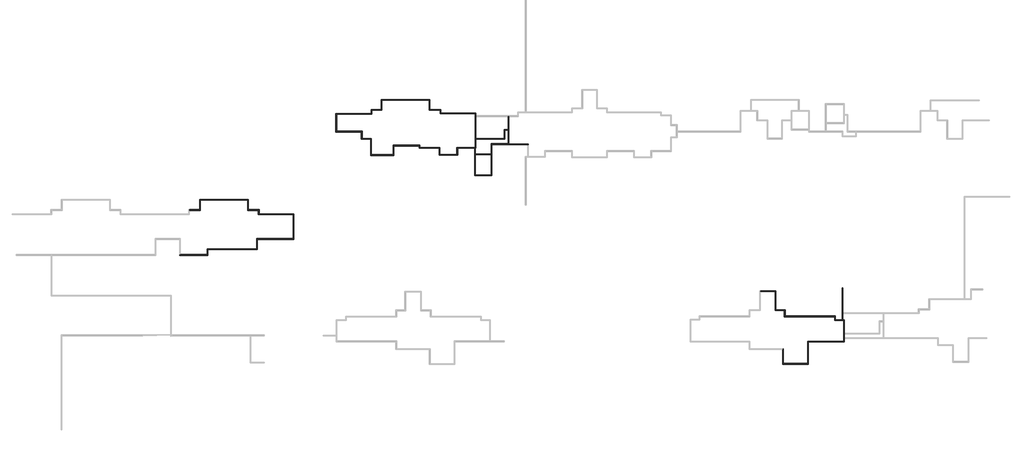
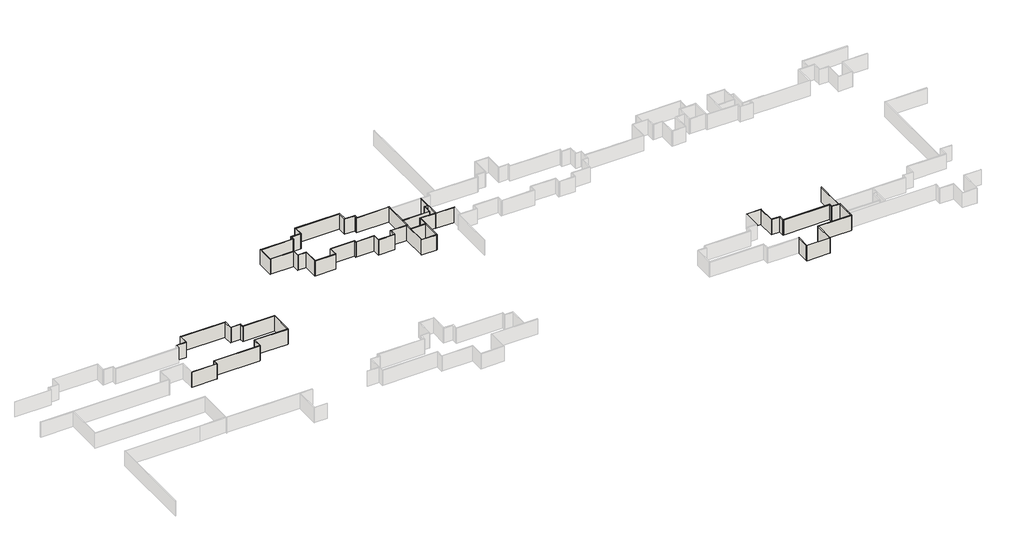
# One storey, part 3 of 8: 60 walls.
"""IFC4 building model written with IfcOpenShell, lengths in millimetres."""

import ifcopenshell
import ifcopenshell.guid

model = None  # the IFC model being written
_history = None  # IfcOwnerHistory: only IFC2X3 demands one
_inside = {}  # id of a spatial element -> (the spatial element, [elements in it])
_under = {}  # id of a project, library or spatial element -> (it, [spatial elements below it])
_declared = {}  # id of a project -> (the project, [libraries it declares])
_typed = {}  # id of a type object -> (the type object, [elements of that type])
_made_of = {}  # id of a material, layer set ... -> (it, [elements and type objects made of it])


def new_model(schema):
    """Start an empty IFC model of exactly this schema.

    Asked for "IFC4X3", IfcOpenShell would pick the latest addendum, in which some entities
    have other attributes; the version numbers below select the first issue.
    IFC2X3 requires an IfcOwnerHistory on every rooted entity: one is made here for all.
    """
    global model, _history
    if schema == "IFC4X3":
        model = ifcopenshell.file(schema_version=(4, 3, 0, 0))
    else:
        model = ifcopenshell.file(schema=schema)
    _inside.clear()
    _under.clear()
    _declared.clear()
    _typed.clear()
    _made_of.clear()
    _history = None
    if model.schema == "IFC2X3":
        org = make("IfcOrganization", Name="unknown")
        user = make(
            "IfcPersonAndOrganization",
            ThePerson=make("IfcPerson", FamilyName="unknown"),
            TheOrganization=org,
        )
        app = make(
            "IfcApplication",
            ApplicationDeveloper=org,
            Version="unknown",
            ApplicationFullName="unknown",
            ApplicationIdentifier="unknown",
        )
        _history = make(
            "IfcOwnerHistory",
            OwningUser=user,
            OwningApplication=app,
            ChangeAction="ADDED",
            CreationDate=0,
        )
    return model


def make(cls, **values):
    """One entity of the class cls with the attributes given. An attribute that is None is left unset."""
    return model.create_entity(
        cls, **{name: value for name, value in values.items() if value is not None}
    )


def rooted(cls, **values):
    """An entity with a GlobalId (a new one), such as an element, a storey or a relation."""
    return make(cls, GlobalId=ifcopenshell.guid.new(), OwnerHistory=_history, **values)


def si_unit(unit_type, name, prefix=None):
    """IfcSIUnit, for example si_unit("LENGTHUNIT", "METRE", prefix="MILLI")."""
    return make("IfcSIUnit", UnitType=unit_type, Prefix=prefix, Name=name)


def assignment(units):
    """IfcUnitAssignment: the units of a project."""
    return None if units is None else make("IfcUnitAssignment", Units=units)


def point(xyz):
    """IfcCartesianPoint."""
    return None if xyz is None else make("IfcCartesianPoint", Coordinates=xyz)


def direction(xyz):
    """IfcDirection."""
    return None if xyz is None else make("IfcDirection", DirectionRatios=xyz)


def frame(location, z_axis=None, x_axis=None):
    """IfcAxis2Placement3D, a coordinate frame: its origin and axes. An axis left out is left unset."""
    return make(
        "IfcAxis2Placement3D",
        Location=point(location),
        Axis=direction(z_axis),
        RefDirection=direction(x_axis),
    )


def origin():
    """The frame at (0, 0, 0) with its axes left unset."""
    return frame((0.0, 0.0, 0.0))


def origin_with_axes():
    """The frame at (0, 0, 0) with the z axis (0, 0, 1) and the x axis (1, 0, 0) written out."""
    return frame((0.0, 0.0, 0.0), z_axis=(0.0, 0.0, 1.0), x_axis=(1.0, 0.0, 0.0))


def place(relative_to, where):
    """IfcLocalPlacement: puts the frame where relative to a parent placement (None: the world)."""
    return make(
        "IfcLocalPlacement", PlacementRelTo=relative_to, RelativePlacement=where
    )


def context(
    kind, dimensions, precision=None, world=None, true_north=None, identifier=None
):
    """IfcGeometricRepresentationContext, for example the 3D "Model" context."""
    return make(
        "IfcGeometricRepresentationContext",
        ContextIdentifier=identifier,
        ContextType=kind,
        CoordinateSpaceDimension=dimensions,
        Precision=precision,
        WorldCoordinateSystem=world,
        TrueNorth=true_north,
    )


def project(units=None, contexts=None):
    """IfcProject with its units and contexts."""
    return rooted(
        "IfcProject",
        Name="project",
        RepresentationContexts=contexts,
        UnitsInContext=assignment(units),
    )


def spatial(cls, under=None, at=None, **own):
    """A site, building, storey or space (cls), placed at a placement, below another one or the project."""
    s = rooted(cls, ObjectPlacement=at, **own)
    if under is not None:
        _under.setdefault(under.id(), (under, []))[1].append(s)
    return s


def polyline(points):
    """IfcPolyline through the points."""
    return make("IfcPolyline", Points=[point(p) for p in points])


def outline(outer, holes=None, kind="AREA"):
    """IfcArbitraryClosedProfileDef: a profile drawn as a closed curve; with holes, ...WithVoids."""
    if holes is None:
        return make("IfcArbitraryClosedProfileDef", ProfileType=kind, OuterCurve=outer)
    return make(
        "IfcArbitraryProfileDefWithVoids",
        ProfileType=kind,
        OuterCurve=outer,
        InnerCurves=holes,
    )


def extrude(swept, where, along, depth):
    """IfcExtrudedAreaSolid: the profile swept, set in the frame where, extruded along a direction by depth."""
    return make(
        "IfcExtrudedAreaSolid",
        SweptArea=swept,
        Position=where,
        ExtrudedDirection=direction(along),
        Depth=depth,
    )


def faces_of(points, faces, orient=None, outer=None):
    """IfcFace entities. A face is a list of loops; a loop is a list of indices into points, from 0.

    orient and outer hold one flag for each loop. By default every Orientation is true, the
    first loop of a face is its IfcFaceOuterBound and the others are IfcFaceBound.
    """
    made = []
    for i, loops in enumerate(faces):
        bounds = []
        for j, loop in enumerate(loops):
            is_outer = j == 0 if outer is None else outer[i][j]
            bounds.append(
                make(
                    "IfcFaceOuterBound" if is_outer else "IfcFaceBound",
                    Bound=make("IfcPolyLoop", Polygon=[points[k] for k in loop]),
                    Orientation=True if orient is None else orient[i][j],
                )
            )
        made.append(make("IfcFace", Bounds=bounds))
    return made


def faceted_brep(points, faces, orient=None, outer=None, voids=None):
    """IfcFacetedBrep: a solid bounded by flat faces; with voids (closed shells), ...WithVoids."""
    shared = [point(p) for p in points]
    hull = make("IfcClosedShell", CfsFaces=faces_of(shared, faces, orient, outer))
    if voids is None:
        return make("IfcFacetedBrep", Outer=hull)
    return make(
        "IfcFacetedBrepWithVoids",
        Outer=hull,
        Voids=[
            make(cls, CfsFaces=faces_of(shared, fs, o, b)) for cls, fs, o, b in voids
        ],
    )


def shape(context_of_items, identifier, shape_type, items):
    """IfcShapeRepresentation: the items that make up one representation, for example the "Body"."""
    return make(
        "IfcShapeRepresentation",
        ContextOfItems=context_of_items,
        RepresentationIdentifier=identifier,
        RepresentationType=shape_type,
        Items=items,
    )


def made_of(thing, what):
    """Note that an element or type object is made of a material, layer set ...; save() writes the relation."""
    if what is not None:
        _made_of.setdefault(what.id(), (what, []))[1].append(thing)
    return thing


def element(
    cls,
    number,
    at=None,
    inside=None,
    cuts=None,
    type_object=None,
    material=None,
    context=None,
    identifier="Body",
    shape_type=None,
    held_by="IfcProductDefinitionShape",
    body=None,
    shapes=None,
    **own,
):
    """One element of the class cls, such as IfcWall. Its Tag is "e" and its number.

    at: its placement. inside: the storey or other place that contains it. cuts: it is an
    opening in that element (IfcRelVoidsElement). A single representation is given by context,
    identifier, shape_type and body (its items); several are given by shapes. held_by: the class
    of the entity that holds the representations. save() writes the other relations.
    """
    e = rooted(cls, Tag="e%d" % number, ObjectPlacement=at, **own)
    if body is not None:
        shapes = [shape(context, identifier, shape_type, body)]
    if shapes is not None:
        e.Representation = make(held_by, Representations=shapes)
    if inside is not None:
        _inside.setdefault(inside.id(), (inside, []))[1].append(e)
    if cuts is not None:
        rooted(
            "IfcRelVoidsElement", RelatingBuildingElement=cuts, RelatedOpeningElement=e
        )
    if type_object is not None:
        _typed.setdefault(type_object.id(), (type_object, []))[1].append(e)
    return made_of(e, material)


def aggregate(whole, parts):
    """IfcRelAggregates: a whole, such as a stair, and the parts it consists of."""
    return rooted("IfcRelAggregates", RelatingObject=whole, RelatedObjects=parts)


def save(model, path):
    """Write the relations noted so far, then the file.

    IfcRelAggregates (storeys below a building ...), IfcRelContainedInSpatialStructure (elements
    in a storey), IfcRelDefinesByType, IfcRelAssociatesMaterial and IfcRelDeclares: one each for
    every whole, place, type object, material and project.
    """
    for whole, parts in _under.values():
        aggregate(whole, parts)
    for where, things in _inside.values():
        rooted(
            "IfcRelContainedInSpatialStructure",
            RelatedElements=things,
            RelatingStructure=where,
        )
    for kind, things in _typed.values():
        rooted("IfcRelDefinesByType", RelatedObjects=things, RelatingType=kind)
    for what, things in _made_of.values():
        rooted("IfcRelAssociatesMaterial", RelatedObjects=things, RelatingMaterial=what)
    for by, libraries in _declared.values():
        rooted("IfcRelDeclares", RelatingContext=by, RelatedDefinitions=libraries)
    model.write(path)


model = new_model("IFC4")

# Units and contexts
model_context = context("Model", 3, world=origin())
ifc_project = project(units=[si_unit("LENGTHUNIT", "METRE", prefix="MILLI")], contexts=[model_context])

# Site, building, storey
site = spatial("IfcSite", under=ifc_project)
building = spatial("IfcBuilding", under=site)
storey = spatial("IfcBuildingStorey", under=building, Name="户型图", Elevation=0.0)

# Walls
placement = place(None, origin())
element("IfcWall", 1, ObjectType="所有墙体", at=placement, inside=storey, context=model_context, shape_type="Brep", body=[
    faceted_brep([(127910.0897862, 79520.2608397, 0.0), (129959.7629292, 79520.2608397, 0.0), (129959.7629292, 79520.2608397, 3300.0), (127910.0897862, 79520.2608397, 3300.0), (127910.0897862, 79640.2608397, 0.0), (127910.0897862, 79640.2608397, 3300.0), (129839.7629292, 79640.2608397, 3300.0), (129959.7629292, 79640.2608397, 3300.0), (129959.7629292, 79640.2608397, 0.0), (129839.7629292, 79640.2608397, 0.0)], [[[0, 1, 2, 3]], [[4, 5, 6, 7, 8, 9]], [[1, 0, 4, 9, 8]], [[3, 2, 7, 6, 5]], [[0, 3, 5, 4]], [[2, 1, 8, 7]]]),
])
element("IfcWall", 2, ObjectType="所有墙体", at=placement, inside=storey, context=model_context, shape_type="Brep", body=[
    faceted_brep([(129959.7629292, 79640.2608397, 0.0), (129959.7629292, 81522.3565617, 0.0), (129959.7629292, 81642.3565617, 0.0), (129959.7629292, 81642.3565617, 3300.0), (129959.7629292, 81522.3565617, 3300.0), (129959.7629292, 79640.2608397, 3300.0), (129839.7629292, 79640.2608397, 0.0), (129839.7629292, 79640.2608397, 3300.0), (129839.7629292, 81642.3565617, 3300.0), (129839.7629292, 81642.3565617, 0.0)], [[[0, 1, 2, 3, 4, 5]], [[6, 7, 8, 9]], [[2, 1, 0, 6, 9]], [[5, 4, 3, 8, 7]], [[0, 5, 7, 6]], [[3, 2, 9, 8]]]),
])
element("IfcWall", 3, ObjectType="所有墙体", at=placement, inside=storey, context=model_context, shape_type="Brep", body=[
    faceted_brep([(129959.7629292, 81522.3565617, 0.0), (139140.3371507, 81522.3565617, 0.0), (139260.3371507, 81522.3565617, 0.0), (139260.3371507, 81522.3565617, 3300.0), (139140.3371507, 81522.3565617, 3300.0), (129959.7629292, 81522.3565617, 3300.0), (129959.7629292, 81642.3565617, 0.0), (129959.7629292, 81642.3565617, 3300.0), (139260.3371507, 81642.3565617, 3300.0), (139260.3371507, 81642.3565617, 0.0)], [[[0, 1, 2, 3, 4, 5]], [[6, 7, 8, 9]], [[2, 1, 0, 6, 9]], [[5, 4, 3, 8, 7]], [[0, 5, 7, 6]], [[3, 2, 9, 8]]]),
])
element("IfcWall", 4, ObjectType="所有墙体", at=placement, inside=storey, context=model_context, shape_type="Brep", body=[
    faceted_brep([(139140.3371507, 81522.3565617, 0.0), (139140.3371507, 79520.2608397, 0.0), (139140.3371507, 79520.2608397, 3300.0), (139140.3371507, 81522.3565617, 3300.0), (139260.3371507, 81522.3565617, 0.0), (139260.3371507, 81522.3565617, 3300.0), (139260.3371507, 79640.2608397, 3300.0), (139260.3371507, 79520.2608397, 3300.0), (139260.3371507, 79520.2608397, 0.0), (139260.3371507, 79640.2608397, 0.0)], [[[0, 1, 2, 3]], [[4, 5, 6, 7, 8, 9]], [[1, 0, 4, 9, 8]], [[3, 2, 7, 6, 5]], [[0, 3, 5, 4]], [[2, 1, 8, 7]]]),
])
element("IfcWall", 5, ObjectType="所有墙体", at=placement, inside=storey, context=model_context, shape_type="Brep", body=[
    faceted_brep([(139260.3371507, 79520.2608397, 0.0), (141190.12079, 79520.2608397, 0.0), (141310.12079, 79520.2608397, 0.0), (141310.12079, 79520.2608397, 3300.0), (141190.12079, 79520.2608397, 3300.0), (139260.3371507, 79520.2608397, 3300.0), (139260.3371507, 79640.2608397, 0.0), (139260.3371507, 79640.2608397, 3300.0), (141310.12079, 79640.2608397, 3300.0), (141310.12079, 79640.2608397, 0.0)], [[[0, 1, 2, 3, 4, 5]], [[6, 7, 8, 9]], [[2, 1, 0, 6, 9]], [[5, 4, 3, 8, 7]], [[0, 5, 7, 6]], [[3, 2, 9, 8]]]),
])
element("IfcWall", 6, ObjectType="所有墙体", at=placement, inside=storey, context=model_context, shape_type="Brep", body=[
    faceted_brep([(141190.12079, 79520.2608397, 0.0), (141190.12079, 78721.1444171, 0.0), (141190.12079, 78721.1444171, 3300.0), (141190.12079, 79520.2608397, 3300.0), (141310.12079, 79520.2608397, 0.0), (141310.12079, 79520.2608397, 3300.0), (141310.12079, 78841.1444171, 3300.0), (141310.12079, 78721.1444171, 3300.0), (141310.12079, 78721.1444171, 0.0), (141310.12079, 78841.1444171, 0.0)], [[[0, 1, 2, 3]], [[4, 5, 6, 7, 8, 9]], [[1, 0, 4, 9, 8]], [[3, 2, 7, 6, 5]], [[0, 3, 5, 4]], [[2, 1, 8, 7]]]),
])
element("IfcWall", 7, ObjectType="所有墙体", at=placement, inside=storey, context=model_context, shape_type="Brep", body=[
    faceted_brep([(141310.12079, 78721.1444171, 0.0), (147870.12079, 78721.1444171, 0.0), (147990.12079, 78721.1444171, 0.0), (147990.12079, 78721.1444171, 3300.0), (147870.12079, 78721.1444171, 3300.0), (141310.12079, 78721.1444171, 3300.0), (141310.12079, 78841.1444171, 0.0), (141310.12079, 78841.1444171, 3300.0), (147990.12079, 78841.1444171, 3300.0), (147990.12079, 78841.1444171, 0.0)], [[[0, 1, 2, 3, 4, 5]], [[6, 7, 8, 9]], [[2, 1, 0, 6, 9]], [[5, 4, 3, 8, 7]], [[0, 5, 7, 6]], [[3, 2, 9, 8]]]),
])
element("IfcWall", 8, ObjectType="所有墙体", at=placement, inside=storey, context=model_context, shape_type="Brep", body=[
    faceted_brep([(147870.12079, 78721.1444171, 0.0), (147870.12079, 74052.1202767, 0.0), (147870.12079, 73932.1202767, 0.0), (147870.12079, 73932.1202767, 3300.0), (147870.12079, 74052.1202767, 3300.0), (147870.12079, 78721.1444171, 3300.0), (147990.12079, 78721.1444171, 0.0), (147990.12079, 78721.1444171, 3300.0), (147990.12079, 74052.1202767, 3300.0), (147990.12079, 73932.1202767, 3300.0), (147990.12079, 73932.1202767, 2700.0), (147990.12079, 73932.1202767, 0.0)], [[[0, 1, 2, 3, 4, 5]], [[6, 7, 8, 9, 10, 11]], [[2, 1, 0, 6, 11]], [[5, 4, 3, 9, 8, 7]], [[0, 5, 7, 6]], [[3, 2, 11, 10, 9]]]),
])
element("IfcWall", 9, ObjectType="所有墙体", at=placement, inside=storey, context=model_context, shape_type="Brep", body=[
    faceted_brep([(147870.12079, 74052.1202767, 0.0), (140890.165529, 74052.1202767, 0.0), (140890.165529, 74052.1202767, 3300.0), (147870.12079, 74052.1202767, 3300.0), (147870.12079, 73932.1202767, 0.0), (147870.12079, 73932.1202767, 3300.0), (141010.165529, 73932.1202767, 3300.0), (140890.165529, 73932.1202767, 3300.0), (140890.165529, 73932.1202767, 0.0), (141010.165529, 73932.1202767, 0.0)], [[[0, 1, 2, 3]], [[4, 5, 6, 7, 8, 9]], [[1, 0, 4, 9, 8]], [[3, 2, 7, 6, 5]], [[0, 3, 5, 4]], [[2, 1, 8, 7]]]),
])
element("IfcWall", 10, ObjectType="所有墙体", at=placement, inside=storey, context=model_context, shape_type="Brep", body=[
    faceted_brep([(140890.165529, 73932.1202767, 0.0), (140890.165529, 72052.4548583, 0.0), (140890.165529, 71932.4548583, 0.0), (140890.165529, 71932.4548583, 3300.0), (140890.165529, 72052.4548583, 3300.0), (140890.165529, 73932.1202767, 3300.0), (141010.165529, 73932.1202767, 0.0), (141010.165529, 73932.1202767, 3300.0), (141010.165529, 71932.4548583, 3300.0), (141010.165529, 71932.4548583, 0.0)], [[[0, 1, 2, 3, 4, 5]], [[6, 7, 8, 9]], [[2, 1, 0, 6, 9]], [[5, 4, 3, 8, 7]], [[0, 5, 7, 6]], [[3, 2, 9, 8]]]),
])
element("IfcWall", 11, ObjectType="所有墙体", at=placement, inside=storey, context=model_context, shape_type="Brep", body=[
    faceted_brep([(140890.165529, 72052.4548583, 0.0), (131290.162691, 72052.4548583, 0.0), (131290.162691, 72052.4548583, 3300.0), (140890.165529, 72052.4548583, 3300.0), (140890.165529, 71932.4548583, 0.0), (140890.165529, 71932.4548583, 3300.0), (131410.162691, 71932.4548583, 3300.0), (131290.162691, 71932.4548583, 3300.0), (131290.162691, 71932.4548583, 0.0), (131410.162691, 71932.4548583, 0.0)], [[[0, 1, 2, 3]], [[4, 5, 6, 7, 8, 9]], [[1, 0, 4, 9, 8]], [[3, 2, 7, 6, 5]], [[0, 3, 5, 4]], [[2, 1, 8, 7]]]),
])
element("IfcWall", 12, ObjectType="所有墙体", at=placement, inside=storey, context=model_context, shape_type="Brep", body=[
    faceted_brep([(131290.162691, 71932.4548583, 0.0), (131290.162691, 70952.1232979, 0.0), (131290.162691, 70832.1232979, 0.0), (131290.162691, 70832.1232979, 3300.0), (131290.162691, 70952.1232979, 3300.0), (131290.162691, 71932.4548583, 3300.0), (131410.162691, 71932.4548583, 0.0), (131410.162691, 71932.4548583, 3300.0), (131410.162691, 70832.1232979, 3300.0), (131410.162691, 70832.1232979, 0.0)], [[[0, 1, 2, 3, 4, 5]], [[6, 7, 8, 9]], [[2, 1, 0, 6, 9]], [[5, 4, 3, 8, 7]], [[0, 5, 7, 6]], [[3, 2, 9, 8]]]),
])
element("IfcWall", 13, ObjectType="所有墙体", at=placement, inside=storey, context=model_context, shape_type="Brep", body=[
    faceted_brep([(131290.162691, 70952.1232979, 0.0), (126110.2513394, 70952.1232979, 0.0), (125990.2513394, 70952.1232979, 0.0), (125990.2513394, 70952.1232979, 3300.0), (126110.2513394, 70952.1232979, 3300.0), (131290.162691, 70952.1232979, 3300.0), (131290.162691, 70832.1232979, 0.0), (131290.162691, 70832.1232979, 3300.0), (125990.2513394, 70832.1232979, 3300.0), (125990.2513394, 70832.1232979, 0.0)], [[[0, 1, 2, 3, 4, 5]], [[6, 7, 8, 9]], [[2, 1, 0, 6, 9]], [[5, 4, 3, 8, 7]], [[0, 5, 7, 6]], [[3, 2, 9, 8]]]),
])
element("IfcWall", 14, ObjectType="所有墙体", at=placement, inside=storey, context=model_context, shape_type="Brep", body=[
    faceted_brep([(189279.4180303, 97612.4890874, 0.0), (189279.4180303, 95102.0462442, 0.0), (189279.4180303, 94982.0462442, 0.0), (189279.4180303, 92353.7889647, 0.0), (189279.4180303, 92233.7889647, 0.0), (189279.4180303, 92173.7889647, 0.0), (189279.4180303, 92173.7889647, 3300.0), (189279.4180303, 92233.7889647, 3300.0), (189279.4180303, 92353.7889647, 3300.0), (189279.4180303, 94982.0462442, 3300.0), (189279.4180303, 95102.0462442, 3300.0), (189279.4180303, 97612.4890874, 3300.0), (189399.4180303, 97612.4890874, 0.0), (189399.4180303, 97612.4890874, 3300.0), (189399.4180303, 92293.7889647, 3300.0), (189399.4180303, 92173.7889647, 3300.0), (189399.4180303, 92173.7889647, 0.0), (189399.4180303, 92293.7889647, 0.0)], [[[0, 1, 2, 3, 4, 5, 6, 7, 8, 9, 10, 11]], [[12, 13, 14, 15, 16, 17]], [[5, 4, 3, 2, 1, 0, 12, 17, 16]], [[11, 10, 9, 8, 7, 6, 15, 14, 13]], [[6, 5, 16, 15]], [[0, 11, 13, 12]]]),
])
element("IfcWall", 15, ObjectType="所有墙体", at=placement, inside=storey, context=model_context, shape_type="Brep", body=[
    faceted_brep([(189399.4180303, 92173.7889647, 0.0), (193080.9640604, 92173.7889647, 0.0), (193200.9640604, 92173.7889647, 0.0), (193200.9640604, 92173.7889647, 3300.0), (193080.9640604, 92173.7889647, 3300.0), (189399.4180303, 92173.7889647, 3300.0), (189399.4180303, 92293.7889647, 0.0), (189399.4180303, 92293.7889647, 3300.0), (193200.9640604, 92293.7889647, 3300.0), (193200.9640604, 92293.7889647, 0.0)], [[[0, 1, 2, 3, 4, 5]], [[6, 7, 8, 9]], [[2, 1, 0, 6, 9]], [[5, 4, 3, 8, 7]], [[0, 5, 7, 6]], [[3, 2, 9, 8]]]),
])
element("IfcWall", 16, ObjectType="所有墙体", at=placement, inside=storey, context=model_context, shape_type="Brep", body=[
    faceted_brep([(156127.8219291, 98150.4331897, 0.0), (156127.8219291, 94631.7418551, 0.0), (156127.8219291, 94631.7418551, 3300.0), (156127.8219291, 97931.8352692, 3300.0), (156127.8219291, 98150.4331897, 3300.0), (156127.8219291, 98150.4331897, 2700.0), (156247.8219291, 98150.4331897, 0.0), (156247.8219291, 98150.4331897, 3300.0), (156247.8219291, 98030.4331897, 3300.0), (156247.8219291, 94751.7418551, 3300.0), (156247.8219291, 94631.7418551, 3300.0), (156247.8219291, 94631.7418551, 0.0), (156247.8219291, 94751.7418551, 0.0), (156247.8219291, 98030.4331897, 0.0), (156179.085005, 98150.4331897, 3300.0)], [[[0, 1, 2, 3, 4, 5]], [[6, 7, 8, 9, 10, 11, 12, 13]], [[1, 0, 6, 13, 12, 11]], [[4, 3, 2, 10, 9, 8, 7, 14]], [[2, 1, 11, 10]], [[0, 5, 4, 14, 7, 6]]]),
])
element("IfcWall", 17, ObjectType="所有墙体", at=placement, inside=storey, context=model_context, shape_type="Brep", body=[
    faceted_brep([(156247.8219291, 94631.7418551, 0.0), (161040.4072035, 94631.7418551, 0.0), (161160.4072035, 94631.7418551, 0.0), (161160.4072035, 94631.7418551, 3300.0), (161040.4072035, 94631.7418551, 3300.0), (156247.8219291, 94631.7418551, 3300.0), (156247.8219291, 94751.7418551, 0.0), (156247.8219291, 94751.7418551, 3300.0), (161160.4072035, 94751.7418551, 3300.0), (161160.4072035, 94751.7418551, 0.0)], [[[0, 1, 2, 3, 4, 5]], [[6, 7, 8, 9]], [[2, 1, 0, 6, 9]], [[5, 4, 3, 8, 7]], [[0, 5, 7, 6]], [[3, 2, 9, 8]]]),
])
element("IfcWall", 18, ObjectType="所有墙体", at=placement, inside=storey, context=model_context, shape_type="Brep", body=[
    faceted_brep([(161040.4072035, 94631.7418551, 0.0), (161040.4072035, 93231.7511932, 0.0), (161040.4072035, 93231.7511932, 3300.0), (161040.4072035, 94631.7418551, 3300.0), (161160.4072035, 94631.7418551, 0.0), (161160.4072035, 94631.7418551, 3300.0), (161160.4072035, 93351.7511932, 3300.0), (161160.4072035, 93231.7511932, 3300.0), (161160.4072035, 93231.7511932, 0.0), (161160.4072035, 93351.7511932, 0.0)], [[[0, 1, 2, 3]], [[4, 5, 6, 7, 8, 9]], [[1, 0, 4, 9, 8]], [[3, 2, 7, 6, 5]], [[0, 3, 5, 4]], [[2, 1, 8, 7]]]),
])
element("IfcWall", 19, ObjectType="所有墙体", at=placement, inside=storey, context=model_context, shape_type="Brep", body=[
    faceted_brep([(161160.4072035, 93231.7511932, 0.0), (162840.4072033, 93231.7511932, 0.0), (162960.4072033, 93231.7511932, 0.0), (162960.4072033, 93231.7511932, 3300.0), (162840.4072033, 93231.7511932, 3300.0), (161160.4072035, 93231.7511932, 3300.0), (161160.4072035, 93351.7511932, 0.0), (161160.4072035, 93351.7511932, 3300.0), (162960.4072033, 93351.7511932, 3300.0), (162960.4072033, 93351.7511932, 0.0)], [[[0, 1, 2, 3, 4, 5]], [[6, 7, 8, 9]], [[2, 1, 0, 6, 9]], [[5, 4, 3, 8, 7]], [[0, 5, 7, 6]], [[3, 2, 9, 8]]]),
])
element("IfcWall", 20, ObjectType="所有墙体", at=placement, inside=storey, context=model_context, shape_type="Brep", body=[
    faceted_brep([(162840.4072033, 93231.7511932, 0.0), (162840.4072033, 90105.9609607, 0.0), (162840.4072033, 90105.9609607, 3300.0), (162840.4072033, 93231.7511932, 3300.0), (162960.4072033, 93231.7511932, 0.0), (162960.4072033, 93231.7511932, 3300.0), (162960.4072033, 90225.9609607, 3300.0), (162960.4072033, 90105.9609607, 3300.0), (162960.4072033, 90105.9609607, 0.0), (162960.4072033, 90225.9609607, 0.0)], [[[0, 1, 2, 3]], [[4, 5, 6, 7, 8, 9]], [[1, 0, 4, 9, 8]], [[3, 2, 7, 6, 5]], [[0, 3, 5, 4]], [[2, 1, 8, 7]]]),
])
element("IfcWall", 21, ObjectType="所有墙体", at=placement, inside=storey, context=model_context, shape_type="Brep", body=[
    faceted_brep([(162960.4072033, 90105.9609607, 0.0), (167260.4072033, 90105.9609607, 0.0), (167260.4072033, 90105.9609607, 2700.0), (167260.4072033, 90105.9609607, 3300.0), (167100.4392887, 90105.9609607, 3300.0), (162960.4072033, 90105.9609607, 3300.0), (162960.4072033, 90225.9609607, 0.0), (162960.4072033, 90225.9609607, 3300.0), (167100.4392887, 90225.9609607, 3300.0), (167140.4072033, 90225.9609607, 3300.0), (167260.4072033, 90225.9609607, 3300.0), (167260.4072033, 90225.9609607, 0.0), (167140.4072033, 90225.9609607, 0.0)], [[[0, 1, 2, 3, 4, 5]], [[6, 7, 8, 9, 10, 11, 12]], [[1, 0, 6, 12, 11]], [[5, 4, 3, 10, 9, 8, 7]], [[0, 5, 7, 6]], [[3, 2, 1, 11, 10]]]),
])
element("IfcWall", 22, ObjectType="所有墙体", at=placement, inside=storey, context=model_context, shape_type="Brep", body=[
    faceted_brep([(167260.4072033, 90225.9609607, 0.0), (167260.4072033, 91931.7511932, 0.0), (167260.4072033, 92051.7511932, 0.0), (167260.4072033, 92051.7511932, 3300.0), (167260.4072033, 91931.7511932, 3300.0), (167260.4072033, 90341.7511932, 3300.0), (167260.4072033, 90225.9609607, 3300.0), (167140.4072033, 90225.9609607, 0.0), (167140.4072033, 90225.9609607, 2700.0), (167140.4072033, 90225.9609607, 3300.0), (167140.4072033, 90341.7511932, 3300.0), (167140.4072033, 92051.7511932, 3300.0), (167140.4072033, 92051.7511932, 0.0)], [[[0, 1, 2, 3, 4, 5, 6]], [[7, 8, 9, 10, 11, 12]], [[2, 1, 0, 7, 12]], [[6, 5, 4, 3, 11, 10, 9]], [[0, 6, 9, 8, 7]], [[3, 2, 12, 11]]]),
])
element("IfcWall", 23, ObjectType="所有墙体", at=placement, inside=storey, context=model_context, shape_type="Brep", body=[
    faceted_brep([(167260.4072033, 91931.7511932, 0.0), (172190.4075168, 91931.7511932, 0.0), (172310.4075168, 91931.7511932, 0.0), (172310.4075168, 91931.7511932, 3300.0), (172190.4075168, 91931.7511932, 3300.0), (167260.4072033, 91931.7511932, 3300.0), (167260.4072033, 92051.7511932, 0.0), (167260.4072033, 92051.7511932, 3300.0), (172310.4075168, 92051.7511932, 3300.0), (172310.4075168, 92051.7511932, 0.0)], [[[0, 1, 2, 3, 4, 5]], [[6, 7, 8, 9]], [[2, 1, 0, 6, 9]], [[5, 4, 3, 8, 7]], [[0, 5, 7, 6]], [[3, 2, 9, 8]]]),
])
element("IfcWall", 24, ObjectType="所有墙体", at=placement, inside=storey, context=model_context, shape_type="Brep", body=[
    faceted_brep([(172190.4075168, 91931.7511932, 0.0), (172190.4075168, 91531.3826392, 0.0), (172190.4075168, 91531.3826392, 3300.0), (172190.4075168, 91931.7511932, 3300.0), (172310.4075168, 91931.7511932, 0.0), (172310.4075168, 91931.7511932, 3300.0), (172310.4075168, 91651.3826392, 3300.0), (172310.4075168, 91531.3826392, 3300.0), (172310.4075168, 91531.3826392, 0.0), (172310.4075168, 91651.3826392, 0.0)], [[[0, 1, 2, 3]], [[4, 5, 6, 7, 8, 9]], [[1, 0, 4, 9, 8]], [[3, 2, 7, 6, 5]], [[0, 3, 5, 4]], [[2, 1, 8, 7]]]),
])
element("IfcWall", 25, ObjectType="所有墙体", at=placement, inside=storey, context=model_context, shape_type="Brep", body=[
    faceted_brep([(172310.4075168, 91531.3826392, 0.0), (176040.4072033, 91531.3826392, 0.0), (176160.4072033, 91531.3826392, 0.0), (176160.4072033, 91531.3826392, 3300.0), (176040.4072033, 91531.3826392, 3300.0), (172310.4075168, 91531.3826392, 3300.0), (172310.4075168, 91651.3826392, 0.0), (172310.4075168, 91651.3826392, 3300.0), (176160.4072033, 91651.3826392, 3300.0), (176160.4072033, 91651.3826392, 0.0)], [[[0, 1, 2, 3, 4, 5]], [[6, 7, 8, 9]], [[2, 1, 0, 6, 9]], [[5, 4, 3, 8, 7]], [[0, 5, 7, 6]], [[3, 2, 9, 8]]]),
])
element("IfcWall", 26, ObjectType="所有墙体", at=placement, inside=storey, context=model_context, shape_type="Brep", body=[
    faceted_brep([(176040.4072033, 91531.3826392, 0.0), (176040.4072033, 90131.7511932, 0.0), (176040.4072033, 90131.7511932, 3300.0), (176040.4072033, 91531.3826392, 3300.0), (176160.4072033, 91531.3826392, 0.0), (176160.4072033, 91531.3826392, 3300.0), (176160.4072033, 90251.7511932, 3300.0), (176160.4072033, 90131.7511932, 3300.0), (176160.4072033, 90131.7511932, 0.0), (176160.4072033, 90251.7511932, 0.0)], [[[0, 1, 2, 3]], [[4, 5, 6, 7, 8, 9]], [[1, 0, 4, 9, 8]], [[3, 2, 7, 6, 5]], [[0, 3, 5, 4]], [[2, 1, 8, 7]]]),
])
element("IfcWall", 27, ObjectType="所有墙体", at=placement, inside=storey, context=model_context, shape_type="Brep", body=[
    faceted_brep([(176160.4072033, 90131.7511932, 0.0), (179560.4072033, 90131.7511932, 0.0), (179560.4072033, 90131.7511932, 3300.0), (176160.4072033, 90131.7511932, 3300.0), (176160.4072033, 90251.7511932, 0.0), (176160.4072033, 90251.7511932, 3300.0), (179440.4072033, 90251.7511932, 3300.0), (179560.4072033, 90251.7511932, 3300.0), (179560.4072033, 90251.7511932, 0.0), (179440.4072033, 90251.7511932, 0.0)], [[[0, 1, 2, 3]], [[4, 5, 6, 7, 8, 9]], [[1, 0, 4, 9, 8]], [[3, 2, 7, 6, 5]], [[0, 3, 5, 4]], [[2, 1, 8, 7]]]),
])
element("IfcWall", 28, ObjectType="所有墙体", at=placement, inside=storey, context=model_context, shape_type="Brep", body=[
    faceted_brep([(179560.4072033, 90251.7511932, 0.0), (179560.4072033, 91531.3826392, 0.0), (179560.4072033, 91651.3826392, 0.0), (179560.4072033, 91651.3826392, 3300.0), (179560.4072033, 91531.3826392, 3300.0), (179560.4072033, 90251.7511932, 3300.0), (179440.4072033, 90251.7511932, 0.0), (179440.4072033, 90251.7511932, 3300.0), (179440.4072033, 91651.3826392, 3300.0), (179440.4072033, 91651.3826392, 0.0)], [[[0, 1, 2, 3, 4, 5]], [[6, 7, 8, 9]], [[2, 1, 0, 6, 9]], [[5, 4, 3, 8, 7]], [[0, 5, 7, 6]], [[3, 2, 9, 8]]]),
])
element("IfcWall", 29, ObjectType="所有墙体", at=placement, inside=storey, context=model_context, shape_type="Brep", body=[
    faceted_brep([(179560.4072033, 91531.3826392, 0.0), (182840.4077224, 91531.3826392, 0.0), (182960.4077224, 91531.3826392, 0.0), (183060.4077201, 91531.3826392, 0.0), (183060.4077201, 91531.3826392, 3300.0), (182960.4077224, 91531.3826392, 3300.0), (182840.4077224, 91531.3826392, 3300.0), (179560.4072033, 91531.3826392, 3300.0), (179560.4072033, 91651.3826392, 0.0), (179560.4072033, 91651.3826392, 3300.0), (182940.4077201, 91651.3826392, 3300.0), (183060.4077201, 91651.3826392, 3300.0), (183060.4077201, 91651.3826392, 0.0), (182940.4077201, 91651.3826392, 0.0)], [[[0, 1, 2, 3, 4, 5, 6, 7]], [[8, 9, 10, 11, 12, 13]], [[3, 2, 1, 0, 8, 13, 12]], [[7, 6, 5, 4, 11, 10, 9]], [[0, 7, 9, 8]], [[4, 3, 12, 11]]]),
])
element("IfcWall", 30, ObjectType="所有墙体", at=placement, inside=storey, context=model_context, shape_type="Brep", body=[
    faceted_brep([(183060.4077201, 91651.3826392, 0.0), (183060.4077201, 93231.7450908, 0.0), (183060.4077201, 93351.7450908, 0.0), (183060.4077201, 97612.4890874, 0.0), (183060.4077201, 97732.4890874, 0.0), (183060.4077201, 98250.4331897, 0.0), (183060.4077201, 98250.4331897, 3300.0), (183060.4077201, 97732.4890874, 3300.0), (183060.4077201, 97612.4890874, 3300.0), (183060.4077201, 93351.7450908, 3300.0), (183060.4077201, 93231.7450908, 3300.0), (183060.4077201, 91651.3826392, 3300.0), (182940.4077201, 91651.3826392, 0.0), (182940.4077201, 91651.3826392, 3300.0), (182940.4077201, 98130.4331897, 3300.0), (182940.4077201, 98250.4331897, 3300.0), (182940.4077201, 98250.4331897, 0.0), (182940.4077201, 98130.4331897, 0.0)], [[[0, 1, 2, 3, 4, 5, 6, 7, 8, 9, 10, 11]], [[12, 13, 14, 15, 16, 17]], [[5, 4, 3, 2, 1, 0, 12, 17, 16]], [[11, 10, 9, 8, 7, 6, 15, 14, 13]], [[0, 11, 13, 12]], [[6, 5, 16, 15]]]),
])
element("IfcWall", 31, ObjectType="所有墙体", at=placement, inside=storey, context=model_context, shape_type="Brep", body=[
    faceted_brep([(182940.4077201, 98250.4331897, 0.0), (176349.86269, 98250.4331897, 0.0), (176229.86269, 98250.4331897, 0.0), (176229.86269, 98250.4331897, 3300.0), (176349.86269, 98250.4331897, 3300.0), (182940.4077201, 98250.4331897, 3300.0), (182940.4077201, 98130.4331897, 0.0), (182940.4077201, 98130.4331897, 3300.0), (176229.86269, 98130.4331897, 3300.0), (176229.86269, 98130.4331897, 0.0)], [[[0, 1, 2, 3, 4, 5]], [[6, 7, 8, 9]], [[2, 1, 0, 6, 9]], [[5, 4, 3, 8, 7]], [[0, 5, 7, 6]], [[3, 2, 9, 8]]]),
])
element("IfcWall", 32, ObjectType="所有墙体", at=placement, inside=storey, context=model_context, shape_type="Brep", body=[
    faceted_brep([(176349.86269, 98250.4331897, 0.0), (176349.86269, 98950.4331897, 0.0), (176349.86269, 98950.4331897, 3300.0), (176349.86269, 98250.4331897, 3300.0), (176229.86269, 98250.4331897, 0.0), (176229.86269, 98250.4331897, 3300.0), (176229.86269, 98830.4331897, 3300.0), (176229.86269, 98950.4331897, 3300.0), (176229.86269, 98950.4331897, 0.0), (176229.86269, 98830.4331897, 0.0)], [[[0, 1, 2, 3]], [[4, 5, 6, 7, 8, 9]], [[1, 0, 4, 9, 8]], [[3, 2, 7, 6, 5]], [[0, 3, 5, 4]], [[2, 1, 8, 7]]]),
])
element("IfcWall", 33, ObjectType="所有墙体", at=placement, inside=storey, context=model_context, shape_type="Brep", body=[
    faceted_brep([(176229.86269, 98950.4331897, 0.0), (174249.8870953, 98950.4331897, 0.0), (174129.8870953, 98950.4331897, 0.0), (174129.8870953, 98950.4331897, 3300.0), (174249.8870953, 98950.4331897, 3300.0), (176229.86269, 98950.4331897, 3300.0), (176229.86269, 98830.4331897, 0.0), (176229.86269, 98830.4331897, 3300.0), (174129.8870953, 98830.4331897, 3300.0), (174129.8870953, 98830.4331897, 0.0)], [[[0, 1, 2, 3, 4, 5]], [[6, 7, 8, 9]], [[2, 1, 0, 6, 9]], [[5, 4, 3, 8, 7]], [[0, 5, 7, 6]], [[3, 2, 9, 8]]]),
])
element("IfcWall", 34, ObjectType="所有墙体", at=placement, inside=storey, context=model_context, shape_type="Brep", body=[
    faceted_brep([(174249.8870953, 98950.4331897, 0.0), (174249.8870953, 100902.3018651, 0.0), (174249.8870953, 100902.3018651, 3300.0), (174249.8870953, 98950.4331897, 3300.0), (174129.8870953, 98950.4331897, 0.0), (174129.8870953, 98950.4331897, 3300.0), (174129.8870953, 100782.3018651, 3300.0), (174129.8870953, 100902.3018651, 3300.0), (174129.8870953, 100902.3018651, 0.0), (174129.8870953, 100782.3018651, 0.0)], [[[0, 1, 2, 3]], [[4, 5, 6, 7, 8, 9]], [[1, 0, 4, 9, 8]], [[3, 2, 7, 6, 5]], [[0, 3, 5, 4]], [[2, 1, 8, 7]]]),
])
element("IfcWall", 35, ObjectType="所有墙体", at=placement, inside=storey, context=model_context, shape_type="Brep", body=[
    faceted_brep([(174129.8870953, 100902.3018651, 0.0), (164879.9002964, 100902.3018651, 0.0), (164879.9002964, 100902.3018651, 3300.0), (174129.8870953, 100902.3018651, 3300.0), (174129.8870953, 100782.3018651, 0.0), (174129.8870953, 100782.3018651, 3300.0), (164999.9002964, 100782.3018651, 3300.0), (164879.9002964, 100782.3018651, 3300.0), (164879.9002964, 100782.3018651, 0.0), (164999.9002964, 100782.3018651, 0.0)], [[[0, 1, 2, 3]], [[4, 5, 6, 7, 8, 9]], [[1, 0, 4, 9, 8]], [[3, 2, 7, 6, 5]], [[0, 3, 5, 4]], [[2, 1, 8, 7]]]),
])
element("IfcWall", 36, ObjectType="所有墙体", at=placement, inside=storey, context=model_context, shape_type="Brep", body=[
    faceted_brep([(164879.9002964, 100782.3018651, 0.0), (164879.9002964, 98950.4331897, 0.0), (164879.9002964, 98830.4331897, 0.0), (164879.9002964, 98830.4331897, 3300.0), (164879.9002964, 98950.4331897, 3300.0), (164879.9002964, 100782.3018651, 3300.0), (164999.9002964, 100782.3018651, 0.0), (164999.9002964, 100782.3018651, 3300.0), (164999.9002964, 98830.4331897, 3300.0), (164999.9002964, 98830.4331897, 0.0)], [[[0, 1, 2, 3, 4, 5]], [[6, 7, 8, 9]], [[2, 1, 0, 6, 9]], [[5, 4, 3, 8, 7]], [[0, 5, 7, 6]], [[3, 2, 9, 8]]]),
])
element("IfcWall", 37, ObjectType="所有墙体", at=placement, inside=storey, context=model_context, shape_type="Brep", body=[
    faceted_brep([(164879.9002964, 98950.4331897, 0.0), (162917.5304809, 98950.4331897, 0.0), (162917.5304809, 98950.4331897, 3300.0), (164879.9002964, 98950.4331897, 3300.0), (164879.9002964, 98830.4331897, 0.0), (164879.9002964, 98830.4331897, 3300.0), (163037.5304809, 98830.4331897, 3300.0), (162917.5304809, 98830.4331897, 3300.0), (162917.5304809, 98830.4331897, 0.0), (163037.5304809, 98830.4331897, 0.0)], [[[0, 1, 2, 3]], [[4, 5, 6, 7, 8, 9]], [[1, 0, 4, 9, 8]], [[3, 2, 7, 6, 5]], [[0, 3, 5, 4]], [[2, 1, 8, 7]]]),
])
element("IfcWall", 38, ObjectType="所有墙体", at=placement, inside=storey, context=model_context, shape_type="Brep", body=[
    faceted_brep([(162917.5304809, 98830.4331897, 0.0), (162917.5304809, 98150.4331897, 0.0), (162917.5304809, 98030.4331897, 0.0), (162917.5304809, 98030.4331897, 3300.0), (162917.5304809, 98150.4331897, 3300.0), (162917.5304809, 98830.4331897, 3300.0), (163037.5304809, 98830.4331897, 0.0), (163037.5304809, 98830.4331897, 3300.0), (163037.5304809, 98030.4331897, 3300.0), (163037.5304809, 98030.4331897, 0.0)], [[[0, 1, 2, 3, 4, 5]], [[6, 7, 8, 9]], [[2, 1, 0, 6, 9]], [[5, 4, 3, 8, 7]], [[0, 5, 7, 6]], [[3, 2, 9, 8]]]),
])
element("IfcWall", 39, ObjectType="所有墙体", at=placement, inside=storey, context=model_context, shape_type="SweptSolid", body=[
    extrude(outline(polyline([(156247.8219291, 98150.4331897), (162917.5304809, 98150.4331897), (162917.5304809, 98030.4331897), (156247.8219291, 98030.4331897), (156247.8219291, 98150.4331897)])), origin_with_axes(), (0.0, 0.0, 1.0), 3300.0),
])
element("IfcWall", 40, ObjectType="所有墙体", at=placement, inside=storey, context=model_context, shape_type="Brep", body=[
    faceted_brep([(189279.4180303, 95102.0462442, 0.0), (188540.4072025, 95102.0462442, 0.0), (188540.4072025, 95102.0462442, 3300.0), (189279.4180303, 95102.0462442, 3300.0), (189279.4180303, 94982.0462442, 0.0), (189279.4180303, 94982.0462442, 3300.0), (188660.4072025, 94982.0462442, 3300.0), (188540.4072025, 94982.0462442, 3300.0), (188540.4072025, 94982.0462442, 0.0), (188660.4072025, 94982.0462442, 0.0)], [[[0, 1, 2, 3]], [[4, 5, 6, 7, 8, 9]], [[1, 0, 4, 9, 8]], [[3, 2, 7, 6, 5]], [[0, 3, 5, 4]], [[2, 1, 8, 7]]]),
])
element("IfcWall", 41, ObjectType="所有墙体", at=placement, inside=storey, context=model_context, shape_type="Brep", body=[
    faceted_brep([(188540.4072025, 94982.0462442, 0.0), (188540.4072025, 93351.7450908, 0.0), (188540.4072025, 93231.7450908, 0.0), (188540.4072025, 93231.7450908, 3300.0), (188540.4072025, 93351.7450908, 3300.0), (188540.4072025, 94982.0462442, 3300.0), (188660.4072025, 94982.0462442, 0.0), (188660.4072025, 94982.0462442, 3300.0), (188660.4072025, 93231.7450908, 3300.0), (188660.4072025, 93231.7450908, 0.0)], [[[0, 1, 2, 3, 4, 5]], [[6, 7, 8, 9]], [[2, 1, 0, 6, 9]], [[5, 4, 3, 8, 7]], [[0, 5, 7, 6]], [[3, 2, 9, 8]]]),
])
element("IfcWall", 42, ObjectType="所有墙体", at=placement, inside=storey, context=model_context, shape_type="SweptSolid", body=[
    extrude(outline(polyline([(183060.4077201, 93351.7450908), (188540.4072025, 93351.7450908), (188540.4072025, 93231.7450908), (183060.4077201, 93231.7450908), (183060.4077201, 93351.7450908)])), origin_with_axes(), (0.0, 0.0, 1.0), 3300.0),
])
element("IfcWall", 43, ObjectType="所有墙体", at=placement, inside=storey, context=model_context, shape_type="Brep", body=[
    faceted_brep([(182840.4077224, 91531.3826392, 0.0), (182840.4077224, 86352.1684203, 0.0), (182840.4077224, 86352.1684203, 3300.0), (182840.4077224, 91531.3826392, 3300.0), (182960.4077224, 91531.3826392, 0.0), (182960.4077224, 91531.3826392, 3300.0), (182960.4077224, 90351.743349, 3300.0), (182960.4077224, 90231.743349, 3300.0), (182960.4077224, 86352.1684203, 3300.0), (182960.4077224, 86352.1684203, 0.0), (182960.4077224, 90231.743349, 0.0), (182960.4077224, 90351.743349, 0.0)], [[[0, 1, 2, 3]], [[4, 5, 6, 7, 8, 9, 10, 11]], [[1, 0, 4, 11, 10, 9]], [[3, 2, 8, 7, 6, 5]], [[0, 3, 5, 4]], [[2, 1, 9, 8]]]),
])
element("IfcWall", 44, ObjectType="所有墙体", at=placement, inside=storey, context=model_context, shape_type="SweptSolid", body=[
    extrude(outline(polyline([(186040.4077224, 90231.743349), (182960.4077224, 90231.743349), (182960.4077224, 90351.743349), (186040.4077224, 90351.743349), (186040.4077224, 90231.743349)])), origin_with_axes(), (0.0, 0.0, 1.0), 3300.0),
])
element("IfcWall", 45, ObjectType="所有墙体", at=placement, inside=storey, context=model_context, shape_type="Brep", body=[
    faceted_brep([(186040.4077224, 92233.7889647, 0.0), (186040.4077224, 90351.743349, 0.0), (186040.4077224, 90231.743349, 0.0), (186040.4077224, 86352.1684203, 0.0), (186040.4077224, 86232.1684203, 0.0), (186040.4077224, 86232.1684203, 3300.0), (186040.4077224, 86352.1684203, 3300.0), (186040.4077224, 86381.1826239, 3300.0), (186040.4077224, 86681.1826239, 3300.0), (186040.4077224, 90231.743349, 3300.0), (186040.4077224, 90351.743349, 3300.0), (186040.4077224, 92233.7889647, 3300.0), (186160.4077224, 92233.7889647, 0.0), (186160.4077224, 92233.7889647, 3300.0), (186160.4077224, 86681.1826239, 3300.0), (186160.4077224, 86381.1826239, 3300.0), (186160.4077224, 86232.1684203, 3300.0), (186160.4077224, 86232.1684203, 0.0)], [[[0, 1, 2, 3, 4, 5, 6, 7, 8, 9, 10, 11]], [[12, 13, 14, 15, 16, 17]], [[4, 3, 2, 1, 0, 12, 17]], [[11, 10, 9, 8, 7, 6, 5, 16, 15, 14, 13]], [[5, 4, 17, 16]], [[0, 11, 13, 12]]]),
])
element("IfcWall", 46, ObjectType="所有墙体", at=placement, inside=storey, context=model_context, shape_type="Brep", body=[
    faceted_brep([(186040.4077224, 86352.1684203, 0.0), (182960.4077224, 86352.1684203, 0.0), (182840.4077224, 86352.1684203, 0.0), (182840.4077224, 86352.1684203, 3300.0), (182960.4077224, 86352.1684203, 3300.0), (183014.313141, 86352.1684203, 3300.0), (186040.4077224, 86352.1684203, 3300.0), (186040.4077224, 86232.1684203, 0.0), (186040.4077224, 86232.1684203, 3300.0), (183054.7628482, 86232.1684203, 3300.0), (182840.4077224, 86232.1684203, 3300.0), (182840.4077224, 86232.1684203, 2700.0), (182840.4077224, 86232.1684203, 0.0)], [[[0, 1, 2, 3, 4, 5, 6]], [[7, 8, 9, 10, 11, 12]], [[2, 1, 0, 7, 12]], [[6, 5, 4, 3, 10, 9, 8]], [[0, 6, 8, 7]], [[3, 2, 12, 11, 10]]]),
])
element("IfcWall", 47, ObjectType="所有墙体", at=placement, inside=storey, context=model_context, shape_type="Brep", body=[
    faceted_brep([(189279.4180303, 92353.7889647, 0.0), (186039.4180303, 92353.7889647, 0.0), (186039.4180303, 92353.7889647, 3300.0), (189279.4180303, 92353.7889647, 3300.0), (189279.4180303, 92233.7889647, 0.0), (189279.4180303, 92233.7889647, 3300.0), (186160.4077224, 92233.7889647, 3300.0), (186040.4077224, 92233.7889647, 3300.0), (186039.4180303, 92233.7889647, 3300.0), (186039.4180303, 92233.7889647, 0.0), (186040.4077224, 92233.7889647, 0.0), (186160.4077224, 92233.7889647, 0.0)], [[[0, 1, 2, 3]], [[4, 5, 6, 7, 8, 9, 10, 11]], [[1, 0, 4, 11, 10, 9]], [[2, 1, 9, 8]], [[3, 2, 8, 7, 6, 5]], [[0, 3, 5, 4]]]),
])
element("IfcWall", 48, ObjectType="所有墙体", at=placement, inside=storey, context=model_context, shape_type="Brep", body=[
    faceted_brep([(253989.7167317, 58282.2610502, 0.0), (253989.7167317, 54252.3246977, 0.0), (253989.7167317, 54132.3246977, 0.0), (253989.7167317, 54132.3246977, 3300.0), (253989.7167317, 54252.3246977, 3300.0), (253989.7167317, 58282.2610502, 3300.0), (254109.7167317, 58282.2610502, 0.0), (254109.7167317, 58282.2610502, 3300.0), (254109.7167317, 55802.3681078, 3300.0), (254109.7167317, 55682.3681078, 3300.0), (254109.7167317, 54952.3246977, 3300.0), (254109.7167317, 54832.3246977, 3300.0), (254109.7167317, 54132.3246977, 3300.0), (254109.7167317, 54132.3246977, 0.0), (254109.7167317, 54832.3246977, 0.0), (254109.7167317, 54952.3246977, 0.0), (254109.7167317, 55682.3681078, 0.0), (254109.7167317, 55802.3681078, 0.0)], [[[0, 1, 2, 3, 4, 5]], [[6, 7, 8, 9, 10, 11, 12, 13, 14, 15, 16, 17]], [[2, 1, 0, 6, 17, 16, 15, 14, 13]], [[5, 4, 3, 12, 11, 10, 9, 8, 7]], [[3, 2, 13, 12]], [[0, 5, 7, 6]]]),
])
element("IfcWall", 49, ObjectType="所有墙体", at=placement, inside=storey, context=model_context, shape_type="Brep", body=[
    faceted_brep([(253989.7167317, 54252.3246977, 0.0), (247039.7341687, 54252.3246977, 0.0), (247039.7341687, 54252.3246977, 3300.0), (253950.1342442, 54252.3246977, 3300.0), (253964.038385, 54252.3246977, 3300.0), (253989.7167317, 54252.3246977, 3300.0), (253989.7167317, 54132.3246977, 0.0), (253989.7167317, 54132.3246977, 3300.0), (253940.9964624, 54132.3246977, 3300.0), (247159.7341687, 54132.3246977, 3300.0), (247039.7341687, 54132.3246977, 3300.0), (247039.7341687, 54132.3246977, 0.0), (247159.7341687, 54132.3246977, 0.0)], [[[0, 1, 2, 3, 4, 5]], [[6, 7, 8, 9, 10, 11, 12]], [[1, 0, 6, 12, 11]], [[5, 4, 3, 2, 10, 9, 8, 7]], [[0, 5, 7, 6]], [[2, 1, 11, 10]]]),
])
element("IfcWall", 50, ObjectType="所有墙体", at=placement, inside=storey, context=model_context, shape_type="Brep", body=[
    faceted_brep([(247039.7341687, 54132.3246977, 0.0), (247039.7341687, 49961.7141002, 0.0), (247039.7341687, 49841.7141002, 0.0), (247039.7341687, 49841.7141002, 3300.0), (247039.7341687, 49961.7141002, 3300.0), (247039.7341687, 54132.3246977, 3300.0), (247159.7341687, 54132.3246977, 0.0), (247159.7341687, 54132.3246977, 3300.0), (247159.7341687, 49901.7141002, 3300.0), (247159.7341687, 49841.7141002, 3300.0), (247159.7341687, 49841.7141002, 2700.0), (247159.7341687, 49841.7141002, 0.0)], [[[0, 1, 2, 3, 4, 5]], [[6, 7, 8, 9, 10, 11]], [[2, 1, 0, 6, 11]], [[5, 4, 3, 9, 8, 7]], [[0, 5, 7, 6]], [[3, 2, 11, 10, 9]]]),
])
element("IfcWall", 51, ObjectType="所有墙体", at=placement, inside=storey, context=model_context, shape_type="Brep", body=[
    faceted_brep([(247039.7341687, 49961.7141002, 0.0), (242338.4382799, 49961.7141002, 0.0), (242218.4382799, 49961.7141002, 0.0), (242218.4382799, 49961.7141002, 3300.0), (242338.4382799, 49961.7141002, 3300.0), (247039.7341687, 49961.7141002, 3300.0), (247039.7341687, 49841.7141002, 0.0), (247039.7341687, 49841.7141002, 3300.0), (242265.632488, 49841.7141002, 3300.0), (242218.4382799, 49841.7141002, 3300.0), (242218.4382799, 49841.7141002, 2700.0), (242218.4382799, 49841.7141002, 0.0), (242218.4382799, 49888.8429011, 3300.0)], [[[0, 1, 2, 3, 4, 5]], [[6, 7, 8, 9, 10, 11]], [[2, 1, 0, 6, 11]], [[5, 4, 3, 12, 9, 8, 7]], [[0, 5, 7, 6]], [[3, 2, 11, 10, 9, 12]]]),
])
element("IfcWall", 52, ObjectType="所有墙体", at=placement, inside=storey, context=model_context, shape_type="Brep", body=[
    faceted_brep([(242338.4382799, 49961.7141002, 0.0), (242338.4382799, 52813.0860808, 0.0), (242338.4382799, 52813.0860808, 3300.0), (242338.4382799, 49961.7141002, 3300.0), (242218.4382799, 49961.7141002, 0.0), (242218.4382799, 49961.7141002, 3300.0), (242218.4382799, 52693.0860808, 3300.0), (242218.4382799, 52813.0860808, 3300.0), (242218.4382799, 52813.0860808, 0.0), (242218.4382799, 52693.0860808, 0.0)], [[[0, 1, 2, 3]], [[4, 5, 6, 7, 8, 9]], [[1, 0, 4, 9, 8]], [[3, 2, 7, 6, 5]], [[0, 3, 5, 4]], [[2, 1, 8, 7]]]),
])
element("IfcWall", 53, ObjectType="所有墙体", at=placement, inside=storey, context=model_context, shape_type="Brep", body=[
    faceted_brep([(237859.8021767, 63882.26105, 0.0), (240739.8021767, 63882.26105, 0.0), (240859.8021767, 63882.26105, 0.0), (240859.8021767, 63882.26105, 3300.0), (240739.8021767, 63882.26105, 3300.0), (237859.8021767, 63882.26105, 3300.0), (237859.8021767, 64002.26105, 0.0), (237859.8021767, 64002.26105, 3300.0), (240859.8021767, 64002.26105, 3300.0), (240859.8021767, 64002.26105, 0.0)], [[[0, 1, 2, 3, 4, 5]], [[6, 7, 8, 9]], [[2, 1, 0, 6, 9]], [[5, 4, 3, 8, 7]], [[0, 5, 7, 6]], [[3, 2, 9, 8]]]),
])
element("IfcWall", 54, ObjectType="所有墙体", at=placement, inside=storey, context=model_context, shape_type="Brep", body=[
    faceted_brep([(240739.8021767, 63882.26105, 0.0), (240739.8021767, 60182.2610504, 0.0), (240739.8021767, 60182.2610504, 3300.0), (240739.8021767, 63882.26105, 3300.0), (240859.8021767, 63882.26105, 0.0), (240859.8021767, 63882.26105, 3300.0), (240859.8021767, 60302.2610504, 3300.0), (240859.8021767, 60182.2610504, 3300.0), (240859.8021767, 60182.2610504, 0.0), (240859.8021767, 60302.2610504, 0.0)], [[[0, 1, 2, 3]], [[4, 5, 6, 7, 8, 9]], [[1, 0, 4, 9, 8]], [[3, 2, 7, 6, 5]], [[0, 3, 5, 4]], [[2, 1, 8, 7]]]),
])
element("IfcWall", 55, ObjectType="所有墙体", at=placement, inside=storey, context=model_context, shape_type="Brep", body=[
    faceted_brep([(240859.8021767, 60182.2610504, 0.0), (242539.8021766, 60182.2610504, 0.0), (242659.8021766, 60182.2610504, 0.0), (242659.8021766, 60182.2610504, 3300.0), (242539.8021766, 60182.2610504, 3300.0), (240859.8021767, 60182.2610504, 3300.0), (240859.8021767, 60302.2610504, 0.0), (240859.8021767, 60302.2610504, 3300.0), (242659.8021766, 60302.2610504, 3300.0), (242659.8021766, 60302.2610504, 0.0)], [[[0, 1, 2, 3, 4, 5]], [[6, 7, 8, 9]], [[2, 1, 0, 6, 9]], [[5, 4, 3, 8, 7]], [[0, 5, 7, 6]], [[3, 2, 9, 8]]]),
])
element("IfcWall", 56, ObjectType="所有墙体", at=placement, inside=storey, context=model_context, shape_type="Brep", body=[
    faceted_brep([(242539.8021766, 60182.2610504, 0.0), (242539.8021766, 58982.2610502, 0.0), (242539.8021766, 58982.2610502, 3300.0), (242539.8021766, 60182.2610504, 3300.0), (242659.8021766, 60182.2610504, 0.0), (242659.8021766, 60182.2610504, 3300.0), (242659.8021766, 59102.2610502, 3300.0), (242659.8021766, 58982.2610502, 3300.0), (242659.8021766, 58982.2610502, 0.0), (242659.8021766, 59102.2610502, 0.0)], [[[0, 1, 2, 3]], [[4, 5, 6, 7, 8, 9]], [[1, 0, 4, 9, 8]], [[3, 2, 7, 6, 5]], [[0, 3, 5, 4]], [[2, 1, 8, 7]]]),
])
element("IfcWall", 57, ObjectType="所有墙体", at=placement, inside=storey, context=model_context, shape_type="Brep", body=[
    faceted_brep([(242659.8021766, 58982.2610502, 0.0), (252239.8021765, 58982.2610502, 0.0), (252359.8021765, 58982.2610502, 0.0), (252359.8021765, 58982.2610502, 3300.0), (252239.8021765, 58982.2610502, 3300.0), (242659.8021766, 58982.2610502, 3300.0), (242659.8021766, 59102.2610502, 0.0), (242659.8021766, 59102.2610502, 3300.0), (252359.8021765, 59102.2610502, 3300.0), (252359.8021765, 59102.2610502, 0.0)], [[[0, 1, 2, 3, 4, 5]], [[6, 7, 8, 9]], [[2, 1, 0, 6, 9]], [[5, 4, 3, 8, 7]], [[0, 5, 7, 6]], [[3, 2, 9, 8]]]),
])
element("IfcWall", 58, ObjectType="所有墙体", at=placement, inside=storey, context=model_context, shape_type="Brep", body=[
    faceted_brep([(252239.8021765, 58982.2610502, 0.0), (252239.8021765, 58282.2610502, 0.0), (252239.8021765, 58282.2610502, 3300.0), (252239.8021765, 58982.2610502, 3300.0), (252359.8021765, 58982.2610502, 0.0), (252359.8021765, 58982.2610502, 3300.0), (252359.8021765, 58402.2610502, 3300.0), (252359.8021765, 58282.2610502, 3300.0), (252359.8021765, 58282.2610502, 0.0), (252359.8021765, 58402.2610502, 0.0)], [[[0, 1, 2, 3]], [[4, 5, 6, 7, 8, 9]], [[1, 0, 4, 9, 8]], [[3, 2, 7, 6, 5]], [[0, 3, 5, 4]], [[2, 1, 8, 7]]]),
])
element("IfcWall", 59, ObjectType="所有墙体", at=placement, inside=storey, context=model_context, shape_type="Brep", body=[
    faceted_brep([(252359.8021765, 58282.2610502, 0.0), (253989.7167317, 58282.2610502, 0.0), (254109.7167317, 58282.2610502, 0.0), (254109.7167317, 58282.2610502, 3300.0), (253989.7167317, 58282.2610502, 3300.0), (252359.8021765, 58282.2610502, 3300.0), (252359.8021765, 58402.2610502, 0.0), (252359.8021765, 58402.2610502, 3300.0), (253689.5875713, 58402.2610502, 3300.0), (253809.5875713, 58402.2610502, 3300.0), (254109.7167317, 58402.2610502, 3300.0), (254109.7167317, 58402.2610502, 0.0), (253809.5875713, 58402.2610502, 0.0), (253689.5875713, 58402.2610502, 0.0)], [[[0, 1, 2, 3, 4, 5]], [[6, 7, 8, 9, 10, 11, 12, 13]], [[2, 1, 0, 6, 13, 12, 11]], [[5, 4, 3, 10, 9, 8, 7]], [[0, 5, 7, 6]], [[3, 2, 11, 10]]]),
])
element("IfcWall", 60, ObjectType="所有墙体", at=placement, inside=storey, context=model_context, shape_type="Brep", body=[
    faceted_brep([(253809.5875713, 58402.2610502, 0.0), (253809.5875713, 59584.9975942, 0.0), (253809.5875713, 59704.9975942, 0.0), (253809.5875713, 64542.2610502, 0.0), (253809.5875713, 64542.2610502, 2700.0), (253809.5875713, 64542.2610502, 3300.0), (253809.5875713, 64392.0126466, 3300.0), (253809.5875713, 59704.9975942, 3300.0), (253809.5875713, 59584.9975942, 3300.0), (253809.5875713, 58402.2610502, 3300.0), (253689.5875713, 58402.2610502, 0.0), (253689.5875713, 58402.2610502, 3300.0), (253689.5875713, 64392.0126466, 3300.0), (253689.5875713, 64503.5900308, 3300.0), (253689.5875713, 64542.2610502, 3300.0), (253689.5875713, 64542.2610502, 0.0), (253762.8884968, 64542.2610502, 3300.0)], [[[0, 1, 2, 3, 4, 5, 6, 7, 8, 9]], [[10, 11, 12, 13, 14, 15]], [[3, 2, 1, 0, 10, 15]], [[5, 4, 3, 15, 14, 16]], [[9, 8, 7, 6, 5, 16, 14, 13, 12, 11]], [[0, 9, 11, 10]]]),
])

save(model, "model.ifc")

# Revit data of these elements
# Type "所有墙体"
#   Layers, outside or top first: 120 mm "默认" (function 1)
# Elements 1, 2, 3, 4, 5, 6, 7, 8, 9, 10, 11, 12, 13 (IfcWall, "所有墙体")
#   Top Offset = 0 mm
#   Base Offset = 0 mm
#   wall height = 3300 mm
#   Phase Created = 新构造
#   Base Constraint = 户型图
#   Top Constraint = 层高
#   Materials on its faces: "默认"
# Elements 14, 15, 16, 17, 18, 19, 20, 21, 22, 23, 24, 25, 26, 27, 28, 29, 30, 31, 32, 33, 34, 35, 36, 37, 38, 39, 40, 41, 42, 43, 44, 45, 46, 47, 48, 49, 50, 51, 52, 53, 54, 55, 56, 57, 58, 59, 60 (IfcWall, "所有墙体")
#   Comments = ""
#   Top Offset = 0 mm
#   Base Offset = 0 mm
#   wall height = 3300 mm
#   Phase Created = 新构造
#   Base Constraint = 户型图
#   Top Constraint = 层高
#   Materials on its faces: "默认"
# Materials
#   "默认": class "其他", colour RGB 192 192 192, transparency 0, Cost = 0
